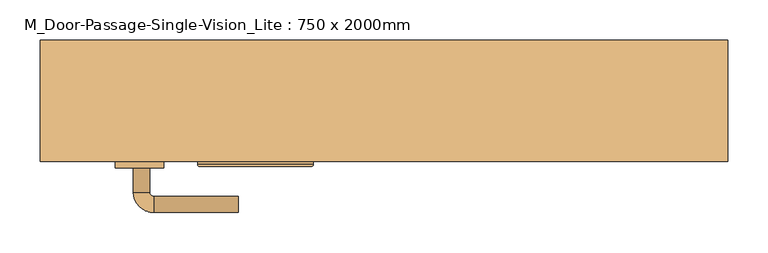
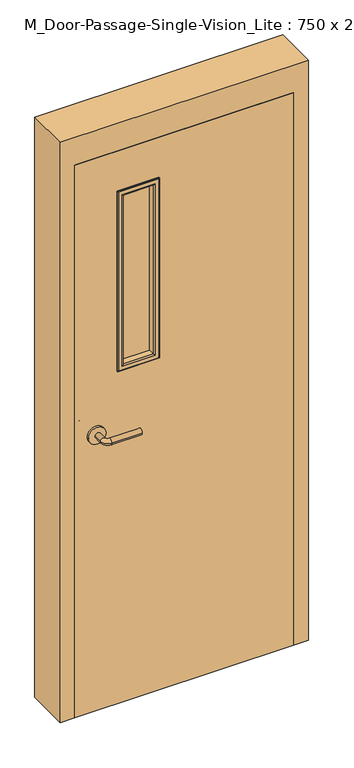
"""IFC4 building model written with IfcOpenShell, lengths in millimetres: door geometry, M_Door-Passage-Single-Vision_Lite : 750 x 2000mm."""

from ifc_helpers import new_model, si_unit, point, frame, frame_2d, origin, place, context, project, spatial, polyline, circle_curve, ellipse_curve, trimmed, segment, composite_curve, outline, extrude, faceted_brep, source, transform, mapped, element, save
from ifc_brep_helpers import plane_surface, cylinder_surface, revolved_surface, advanced_brep


def m_door_passage_single_vision_lite_750_x_2000mm_70ae5a51(model_context):
    return source(origin(), model_context, "Body", "SolidModel", [
        advanced_brep(
        [(-309.990625, -3.35, 1000.0), (-289.990625, -3.35, 1000.0), (-309.990625, 26.65, 1000.0), (-289.990625, 26.65, 1000.0), (-284.990625, 31.65, 1000.0), (-284.990625, 51.65, 1000.0), (-179.990625, 51.65, 1000.0), (-179.990625, 31.65, 1000.0)],
        [
            (0, 1, circle_curve(frame((-299.990625, -3.35, 1000.0), z_axis=(0.0, -1.0, 0.0), x_axis=(1.0, 0.0, 0.0)), 10.0)),
            (1, 0, circle_curve(frame((-299.990625, -3.35, 1000.0), z_axis=(0.0, -1.0, 0.0), x_axis=(1.0, 0.0, 0.0)), 10.0)),
            (0, 2),
            (2, 3, circle_curve(frame((-299.990625, 26.65, 1000.0), z_axis=(0.0, -1.0, 0.0), x_axis=(1.0, 0.0, 0.0)), 10.0)),
            (3, 1),
            (3, 2, circle_curve(frame((-299.990625, 26.65, 1000.0), z_axis=(0.0, -1.0, 0.0), x_axis=(1.0, 0.0, 0.0)), 10.0)),
            (4, 3, circle_curve(frame((-284.990625, 26.65, 1000.0), z_axis=(0.0, 0.0, 1.0), x_axis=(-1.0, 0.0, 0.0)), 5.0)),
            (2, 5, circle_curve(frame((-284.990625, 26.65, 1000.0), z_axis=(0.0, 0.0, -1.0), x_axis=(-1.0, 0.0, 0.0)), 25.0)),
            (5, 4, circle_curve(frame((-284.990625, 41.65, 1000.0), z_axis=(-1.0, 0.0, 0.0), x_axis=(0.0, -1.0, 0.0)), 10.0)),
            (4, 5, circle_curve(frame((-284.990625, 41.65, 1000.0), z_axis=(-1.0, 0.0, 0.0), x_axis=(0.0, -1.0, 0.0)), 10.0)),
            (6, 7, circle_curve(frame((-179.990625, 41.65, 1000.0), z_axis=(1.0, 0.0, 0.0), x_axis=(0.0, -1.0, 0.0)), 10.0)),
            (7, 6, circle_curve(frame((-179.990625, 41.65, 1000.0), z_axis=(1.0, 0.0, 0.0), x_axis=(0.0, -1.0, 0.0)), 10.0)),
            (5, 6),
            (7, 4),
        ],
        [
            plane_surface(frame((-299.990625, -3.35, 1000.0), z_axis=(0.0, -1.0, 0.0), x_axis=(0.0, 0.0, 1.0))),
            cylinder_surface(frame((-299.990625, -3.35, 1000.0), z_axis=(0.0, -1.0, 0.0), x_axis=(1.0, 0.0, 0.0)), 10.0),
            revolved_surface(trimmed(ellipse_curve(frame((-299.990625, 26.65, 1000.0), z_axis=(0.0, -1.0, 0.0), x_axis=(1.0, 0.0, 0.0)), 10.0, 10.0), [point((-309.990625, 26.65, 1000.0))], [point((-289.990625, 26.65, 1000.0))], True, "CARTESIAN"), (-284.990625, 26.65, 1000.0), (0.0, 0.0, -1.0)),
            revolved_surface(trimmed(ellipse_curve(frame((-299.990625, 26.65, 1000.0), z_axis=(0.0, -1.0, 0.0), x_axis=(1.0, 0.0, 0.0)), 10.0, 10.0), [point((-289.990625, 26.65, 1000.0))], [point((-309.990625, 26.65, 1000.0))], True, "CARTESIAN"), (-284.990625, 26.65, 1000.0), (0.0, 0.0, -1.0)),
            plane_surface(frame((-179.990625, 41.65, 1000.0), z_axis=(1.0, 0.0, 0.0), x_axis=(0.0, 0.0, 1.0))),
            cylinder_surface(frame((-284.990625, 41.65, 1000.0), z_axis=(-1.0, 0.0, 0.0), x_axis=(0.0, -1.0, 0.0)), 10.0),
        ],
        [
            (0, [[1, 2]]),
            (1, [[-1, 3, 4, 5]]),
            (1, [[-2, -5, 6, -3]]),
            (2, [[7, -4, 8, 9]]),
            (3, [[-8, -6, -7, 10]]),
            (4, [[11, 12]]),
            (5, [[-9, 13, -12, 14]]),
            (5, [[-10, -14, -11, -13]]),
        ],
    ),
        extrude(outline(composite_curve([segment(trimmed(circle_curve(frame_2d((1000.0, -302.490625)), 30.0), [point((1000.0, -332.490625))], [point((1000.0, -272.490625))], False, "CARTESIAN"), True, "CONTINUOUS"), segment(trimmed(circle_curve(frame_2d((1000.0, -302.490625)), 30.0), [point((1000.0, -272.490625))], [point((1000.0, -332.490625))], False, "CARTESIAN"), True, "CONTINUOUS")], self_intersect=False)), frame((0.0, -11.35, 0.0), z_axis=(0.0, 1.0, 0.0), x_axis=(0.0, 0.0, 1.0)), (0.0, 0.0, 1.0), 8.0),
        advanced_brep(
        [(-309.990625, -64.35, 1000.0), (-289.990625, -64.35, 1000.0), (-289.990625, -94.35, 1000.0), (-309.990625, -94.35, 1000.0), (-284.990625, -99.35, 1000.0), (-284.990625, -119.35, 1000.0), (-179.990625, -119.35, 1000.0), (-179.990625, -99.35, 1000.0)],
        [
            (0, 1, circle_curve(frame((-299.990625, -64.35, 1000.0), z_axis=(0.0, 1.0, 0.0), x_axis=(1.0, 0.0, 0.0)), 10.0)),
            (1, 0, circle_curve(frame((-299.990625, -64.35, 1000.0), z_axis=(0.0, 1.0, 0.0), x_axis=(1.0, 0.0, 0.0)), 10.0)),
            (1, 2),
            (2, 3, circle_curve(frame((-299.990625, -94.35, 1000.0), z_axis=(0.0, 1.0, 0.0), x_axis=(1.0, 0.0, 0.0)), 10.0)),
            (3, 0),
            (3, 2, circle_curve(frame((-299.990625, -94.35, 1000.0), z_axis=(0.0, 1.0, 0.0), x_axis=(1.0, 0.0, 0.0)), 10.0)),
            (4, 5, circle_curve(frame((-284.990625, -109.35, 1000.0), z_axis=(-1.0, 0.0, 0.0), x_axis=(0.0, 1.0, 0.0)), 10.0)),
            (5, 3, circle_curve(frame((-284.990625, -94.35, 1000.0), z_axis=(0.0, 0.0, -1.0), x_axis=(-1.0, 0.0, 0.0)), 25.0)),
            (2, 4, circle_curve(frame((-284.990625, -94.35, 1000.0), z_axis=(0.0, 0.0, 1.0), x_axis=(-1.0, 0.0, 0.0)), 5.0)),
            (5, 4, circle_curve(frame((-284.990625, -109.35, 1000.0), z_axis=(-1.0, 0.0, 0.0), x_axis=(0.0, 1.0, 0.0)), 10.0)),
            (6, 7, circle_curve(frame((-179.990625, -109.35, 1000.0), z_axis=(1.0, 0.0, 0.0), x_axis=(0.0, 1.0, 0.0)), 10.0)),
            (7, 6, circle_curve(frame((-179.990625, -109.35, 1000.0), z_axis=(1.0, 0.0, 0.0), x_axis=(0.0, 1.0, 0.0)), 10.0)),
            (4, 7),
            (6, 5),
        ],
        [
            plane_surface(frame((-299.990625, -64.35, 1000.0), z_axis=(0.0, 1.0, 0.0), x_axis=(0.0, 0.0, 1.0))),
            cylinder_surface(frame((-299.990625, -64.35, 1000.0), z_axis=(0.0, 1.0, 0.0), x_axis=(1.0, 0.0, 0.0)), 10.0),
            revolved_surface(trimmed(ellipse_curve(frame((-299.990625, -94.35, 1000.0), z_axis=(0.0, -1.0, 0.0), x_axis=(1.0, 0.0, 0.0)), 10.0, 10.0), [point((-309.990625, -94.35, 1000.0))], [point((-289.990625, -94.35, 1000.0))], True, "CARTESIAN"), (-284.990625, -94.35, 1000.0), (0.0, 0.0, -1.0)),
            revolved_surface(trimmed(ellipse_curve(frame((-299.990625, -94.35, 1000.0), z_axis=(0.0, -1.0, 0.0), x_axis=(1.0, 0.0, 0.0)), 10.0, 10.0), [point((-289.990625, -94.35, 1000.0))], [point((-309.990625, -94.35, 1000.0))], True, "CARTESIAN"), (-284.990625, -94.35, 1000.0), (0.0, 0.0, -1.0)),
            plane_surface(frame((-179.990625, -109.35, 1000.0), z_axis=(1.0, 0.0, 0.0), x_axis=(0.0, 0.0, 1.0))),
            cylinder_surface(frame((-284.990625, -109.35, 1000.0), z_axis=(-1.0, 0.0, 0.0), x_axis=(0.0, 1.0, 0.0)), 10.0),
        ],
        [
            (0, [[1, 2]]),
            (1, [[3, 4, 5, -2]]),
            (1, [[-5, 6, -3, -1]]),
            (2, [[7, 8, -4, 9]]),
            (3, [[10, -9, -6, -8]]),
            (4, [[11, 12]]),
            (5, [[13, -11, 14, -7]]),
            (5, [[-14, -12, -13, -10]]),
        ],
    ),
        extrude(outline(composite_curve([segment(trimmed(circle_curve(frame_2d((1000.0, -302.490625)), 30.0), [point((1000.0, -332.490625))], [point((1000.0, -272.490625))], False, "CARTESIAN"), True, "CONTINUOUS"), segment(trimmed(circle_curve(frame_2d((1000.0, -302.490625)), 30.0), [point((1000.0, -272.490625))], [point((1000.0, -332.490625))], False, "CARTESIAN"), True, "CONTINUOUS")], self_intersect=False)), frame((0.0, -64.35, 0.0), z_axis=(0.0, 1.0, 0.0), x_axis=(0.0, 0.0, 1.0)), (0.0, 0.0, 1.0), 8.0),
        extrude(outline(polyline([(2000.0, -375.0), (0.0, -375.0), (0.0, 375.0), (2000.0, 375.0), (2000.0, -375.0)]), holes=[polyline([(1847.6, -222.6), (1847.6, -95.6), (1212.6, -95.6), (1212.6, -222.6), (1847.6, -222.6)])]), frame((0.0, -56.35, 0.0), z_axis=(0.0, 1.0, 0.0), x_axis=(0.0, 0.0, 1.0)), (0.0, 0.0, 1.0), 45.0),
        faceted_brep([(375.0, -6.5875, 0.0), (359.125, -6.5875, 0.0), (359.125, 44.4375, 0.0), (375.0, 44.4375, 0.0), (375.0, 93.65, 0.0), (425.0, 93.65, 0.0), (425.0, -56.35, 0.0), (375.0, -56.35, 0.0), (375.0, -56.35, 2000.0), (375.0, -6.5875, 2000.0), (425.0, -56.35, 2100.0), (-425.0, -56.35, 2100.0), (-425.0, -56.35, 0.0), (-375.0, -56.35, 0.0), (-375.0, -56.35, 2000.0), (425.0, 93.65, 2100.0), (375.0, 93.65, 2000.0), (-375.0, 93.65, 2000.0), (-375.0, 93.65, 0.0), (-425.0, 93.65, 0.0), (-425.0, 93.65, 2100.0), (375.0, 44.4375, 2000.0), (359.125, 44.4375, 1984.125), (-359.125, 44.4375, 1984.125), (-359.125, 44.4375, 0.0), (-375.0, 44.4375, 0.0), (-375.0, 44.4375, 2000.0), (359.125, -6.5875, 1984.125), (-375.0, -6.5875, 2000.0), (-375.0, -6.5875, 0.0), (-359.125, -6.5875, 0.0), (-359.125, -6.5875, 1984.125)], [[[0, 1, 2, 3, 4, 5, 6, 7]], [[7, 8, 9, 0]], [[6, 10, 11, 12, 13, 14, 8, 7]], [[5, 15, 10, 6]], [[4, 16, 17, 18, 19, 20, 15, 5]], [[3, 21, 16, 4]], [[2, 22, 23, 24, 25, 26, 21, 3]], [[1, 27, 22, 2]], [[0, 9, 28, 29, 30, 31, 27, 1]], [[8, 14, 28, 9]], [[16, 21, 26, 17]], [[22, 27, 31, 23]], [[12, 19, 18, 25, 24, 30, 29, 13]], [[13, 29, 28, 14]], [[11, 20, 19, 12]], [[17, 26, 25, 18]], [[23, 31, 30, 24]], [[15, 20, 11, 10]]]),
        extrude(outline(polyline([(-95.6, -31.35), (-95.6, -36.35), (-222.6, -36.35), (-222.6, -31.35), (-95.6, -31.35)])), frame((0.0, 0.0, 1212.6), z_axis=(0.0, 0.0, 1.0), x_axis=(1.0, 0.0, 0.0)), (0.0, 0.0, 1.0), 635.0),
        advanced_brep(
        [(-222.6, -36.35, 1847.6), (-222.6, -36.35, 1212.6), (-222.6, -56.35, 1212.6), (-222.6, -56.35, 1847.6), (-210.6, -57.35, 1835.6), (-210.6, -57.35, 1224.6), (-210.6, -36.35, 1224.6), (-210.6, -36.35, 1835.6), (-215.6, -62.35, 1840.6), (-215.6, -62.35, 1219.6), (-230.6, -60.35, 1855.6), (-230.6, -60.35, 1204.6), (-228.6, -62.35, 1206.6), (-228.6, -62.35, 1853.6), (-230.6, -56.35, 1855.6), (-230.6, -56.35, 1204.6), (-95.6, -36.35, 1212.6), (-95.6, -56.35, 1212.6), (-107.6, -57.35, 1224.6), (-107.6, -36.35, 1224.6), (-102.6, -62.35, 1219.6), (-87.6, -60.35, 1204.6), (-89.6, -62.35, 1206.6), (-87.6, -56.35, 1204.6), (-95.6, -36.35, 1847.6), (-95.6, -56.35, 1847.6), (-107.6, -57.35, 1835.6), (-107.6, -36.35, 1835.6), (-102.6, -62.35, 1840.6), (-87.6, -60.35, 1855.6), (-89.6, -62.35, 1853.6), (-87.6, -56.35, 1855.6)],
        [
            (0, 1),
            (1, 2),
            (2, 3),
            (3, 0),
            (4, 5),
            (5, 6),
            (6, 7),
            (7, 4),
            (8, 9),
            (9, 5, ellipse_curve(frame((-215.6, -57.35, 1219.6), z_axis=(-0.7071067811865475, 0.0, 0.7071067811865475), x_axis=(0.7071067811865474, 0.0, 0.7071067811865476)), 7.0710678, 5.0)),
            (4, 8, ellipse_curve(frame((-215.6, -57.35, 1840.6), z_axis=(-0.7071067811865475, 0.0, -0.7071067811865475), x_axis=(-0.7071067811865474, 0.0, 0.7071067811865476)), 7.0710678, 5.0)),
            (10, 11),
            (11, 12, ellipse_curve(frame((-228.6, -60.35, 1206.6), z_axis=(-0.7071067811865475, 0.0, 0.7071067811865475), x_axis=(0.7071067811865474, 0.0, 0.7071067811865476)), 2.8284271, 2.0)),
            (12, 13),
            (13, 10, ellipse_curve(frame((-228.6, -60.35, 1853.6), z_axis=(-0.7071067811865475, 0.0, -0.7071067811865475), x_axis=(-0.7071067811865474, 0.0, 0.7071067811865476)), 2.8284271, 2.0)),
            (14, 15),
            (15, 11),
            (10, 14),
            (1, 16),
            (16, 17),
            (17, 2),
            (5, 18),
            (18, 19),
            (19, 6),
            (9, 20),
            (20, 18, ellipse_curve(frame((-102.6, -57.35, 1219.6), z_axis=(-0.7071067811865475, 0.0, -0.7071067811865475), x_axis=(-0.7071067811865476, 0.0, 0.7071067811865474)), 7.0710678, 5.0)),
            (11, 21),
            (21, 22, ellipse_curve(frame((-89.6, -60.35, 1206.6), z_axis=(-0.7071067811865475, 0.0, -0.7071067811865475), x_axis=(-0.7071067811865476, 0.0, 0.7071067811865474)), 2.8284271, 2.0)),
            (22, 12),
            (15, 23),
            (23, 21),
            (16, 24),
            (24, 25),
            (25, 17),
            (18, 26),
            (26, 27),
            (27, 19),
            (20, 28),
            (28, 26, ellipse_curve(frame((-102.6, -57.35, 1840.6), z_axis=(0.7071067811865475, 0.0, -0.7071067811865475), x_axis=(-0.7071067811865474, 0.0, -0.7071067811865476)), 7.0710678, 5.0)),
            (21, 29),
            (29, 30, ellipse_curve(frame((-89.6, -60.35, 1853.6), z_axis=(0.7071067811865475, 0.0, -0.7071067811865475), x_axis=(-0.7071067811865474, 0.0, -0.7071067811865476)), 2.8284271, 2.0)),
            (30, 22),
            (23, 31),
            (31, 29),
            (14, 31),
            (25, 3),
            (24, 0),
            (27, 7),
            (26, 4),
            (28, 8),
            (30, 13),
            (29, 10),
        ],
        [
            plane_surface(frame((-222.6, -56.35, 1847.6), z_axis=(-1.0, 0.0, 0.0), x_axis=(0.0, 0.0, -1.0))),
            plane_surface(frame((-210.6, -36.35, 1835.6), z_axis=(1.0, 0.0, 0.0), x_axis=(0.0, 0.0, -1.0))),
            cylinder_surface(frame((-215.6, -57.35, 1847.6), z_axis=(0.0, 0.0, 1.0), x_axis=(-1.0, 0.0, 0.0)), 5.0),
            cylinder_surface(frame((-228.6, -60.35, 1847.6), z_axis=(0.0, 0.0, 1.0), x_axis=(-1.0, 0.0, 0.0)), 2.0),
            plane_surface(frame((-230.6, -60.35, 1855.6), z_axis=(-1.0, 0.0, 0.0), x_axis=(0.0, 0.0, -1.0))),
            plane_surface(frame((-222.6, -56.35, 1212.6), z_axis=(0.0, 0.0, -1.0), x_axis=(1.0, 0.0, 0.0))),
            plane_surface(frame((-210.6, -36.35, 1224.6), z_axis=(0.0, 0.0, 1.0), x_axis=(1.0, 0.0, 0.0))),
            cylinder_surface(frame((-222.6, -57.35, 1219.6), z_axis=(-1.0, 0.0, 0.0), x_axis=(0.0, 0.0, -1.0)), 5.0),
            cylinder_surface(frame((-222.6, -60.35, 1206.6), z_axis=(-1.0, 0.0, 0.0), x_axis=(0.0, 0.0, -1.0)), 2.0),
            plane_surface(frame((-230.6, -60.35, 1204.6), z_axis=(0.0, 0.0, -1.0), x_axis=(1.0, 0.0, 0.0))),
            plane_surface(frame((-95.6, -56.35, 1212.6), z_axis=(1.0, 0.0, 0.0), x_axis=(0.0, 0.0, 1.0))),
            plane_surface(frame((-107.6, -36.35, 1224.6), z_axis=(-1.0, 0.0, 0.0), x_axis=(0.0, 0.0, 1.0))),
            cylinder_surface(frame((-102.6, -57.35, 1212.6), z_axis=(0.0, 0.0, -1.0), x_axis=(1.0, 0.0, 0.0)), 5.0),
            cylinder_surface(frame((-89.6, -60.35, 1212.6), z_axis=(0.0, 0.0, -1.0), x_axis=(1.0, 0.0, 0.0)), 2.0),
            plane_surface(frame((-87.6, -60.35, 1204.6), z_axis=(1.0, 0.0, 0.0), x_axis=(0.0, 0.0, 1.0))),
            plane_surface(frame((-87.6, -56.35, 1855.6), z_axis=(0.0, 1.0, 0.0), x_axis=(-1.0, 0.0, 0.0))),
            plane_surface(frame((-95.6, -56.35, 1847.6), z_axis=(0.0, 0.0, 1.0), x_axis=(-1.0, 0.0, 0.0))),
            plane_surface(frame((-95.6, -36.35, 1847.6), z_axis=(0.0, 1.0, 0.0), x_axis=(-1.0, 0.0, 0.0))),
            plane_surface(frame((-107.6, -36.35, 1835.6), z_axis=(0.0, 0.0, -1.0), x_axis=(-1.0, 0.0, 0.0))),
            cylinder_surface(frame((-95.6, -57.35, 1840.6), z_axis=(1.0, 0.0, 0.0), x_axis=(0.0, 0.0, 1.0)), 5.0),
            plane_surface(frame((-102.6, -62.35, 1840.6), z_axis=(0.0, -1.0, 0.0), x_axis=(-1.0, 0.0, 0.0))),
            cylinder_surface(frame((-95.6, -60.35, 1853.6), z_axis=(1.0, 0.0, 0.0), x_axis=(0.0, 0.0, 1.0)), 2.0),
            plane_surface(frame((-87.6, -60.35, 1855.6), z_axis=(0.0, 0.0, 1.0), x_axis=(-1.0, 0.0, 0.0))),
        ],
        [
            (0, [[1, 2, 3, 4]]),
            (1, [[5, 6, 7, 8]]),
            (2, [[9, 10, -5, 11]]),
            (3, [[12, 13, 14, 15]]),
            (4, [[16, 17, -12, 18]]),
            (5, [[19, 20, 21, -2]]),
            (6, [[22, 23, 24, -6]]),
            (7, [[25, 26, -22, -10]]),
            (8, [[27, 28, 29, -13]]),
            (9, [[30, 31, -27, -17]]),
            (10, [[32, 33, 34, -20]]),
            (11, [[35, 36, 37, -23]]),
            (12, [[38, 39, -35, -26]]),
            (13, [[40, 41, 42, -28]]),
            (14, [[43, 44, -40, -31]]),
            (15, [[-16, 45, -43, -30], [-3, -21, -34, 46]]),
            (16, [[47, -4, -46, -33]]),
            (17, [[-1, -47, -32, -19], [-7, -24, -37, 48]]),
            (18, [[49, -8, -48, -36]]),
            (19, [[50, -11, -49, -39]]),
            (20, [[-14, -29, -42, 51], [-9, -50, -38, -25]]),
            (21, [[52, -15, -51, -41]]),
            (22, [[-45, -18, -52, -44]]),
        ],
    ),
        advanced_brep(
        [(-222.6, -31.35, 1212.6), (-222.6, -31.35, 1847.6), (-222.6, -11.35, 1847.6), (-222.6, -11.35, 1212.6), (-210.6, -10.35, 1224.6), (-210.6, -10.35, 1835.6), (-210.6, -31.35, 1835.6), (-210.6, -31.35, 1224.6), (-215.6, -5.35, 1219.6), (-215.6, -5.35, 1840.6), (-230.6, -7.35, 1204.6), (-230.6, -7.35, 1855.6), (-228.6, -5.35, 1853.6), (-228.6, -5.35, 1206.6), (-230.6, -11.35, 1204.6), (-230.6, -11.35, 1855.6), (-95.6, -31.35, 1847.6), (-95.6, -11.35, 1847.6), (-107.6, -10.35, 1835.6), (-107.6, -31.35, 1835.6), (-102.6, -5.35, 1840.6), (-87.6, -7.35, 1855.6), (-89.6, -5.35, 1853.6), (-87.6, -11.35, 1855.6), (-95.6, -31.35, 1212.6), (-95.6, -11.35, 1212.6), (-107.6, -10.35, 1224.6), (-107.6, -31.35, 1224.6), (-102.6, -5.35, 1219.6), (-87.6, -7.35, 1204.6), (-89.6, -5.35, 1206.6), (-87.6, -11.35, 1204.6)],
        [
            (0, 1),
            (1, 2),
            (2, 3),
            (3, 0),
            (4, 5),
            (5, 6),
            (6, 7),
            (7, 4),
            (8, 9),
            (9, 5, ellipse_curve(frame((-215.6, -10.35, 1840.6), z_axis=(-0.7071067811865475, 0.0, -0.7071067811865475), x_axis=(0.7071067811865474, 0.0, -0.7071067811865476)), 7.0710678, 5.0)),
            (4, 8, ellipse_curve(frame((-215.6, -10.35, 1219.6), z_axis=(-0.7071067811865475, 0.0, 0.7071067811865475), x_axis=(-0.7071067811865474, 0.0, -0.7071067811865476)), 7.0710678, 5.0)),
            (10, 11),
            (11, 12, ellipse_curve(frame((-228.6, -7.35, 1853.6), z_axis=(-0.7071067811865475, 0.0, -0.7071067811865475), x_axis=(0.7071067811865474, 0.0, -0.7071067811865476)), 2.8284271, 2.0)),
            (12, 13),
            (13, 10, ellipse_curve(frame((-228.6, -7.35, 1206.6), z_axis=(-0.7071067811865475, 0.0, 0.7071067811865475), x_axis=(-0.7071067811865474, 0.0, -0.7071067811865476)), 2.8284271, 2.0)),
            (14, 15),
            (15, 11),
            (10, 14),
            (1, 16),
            (16, 17),
            (17, 2),
            (5, 18),
            (18, 19),
            (19, 6),
            (9, 20),
            (20, 18, ellipse_curve(frame((-102.6, -10.35, 1840.6), z_axis=(-0.7071067811865475, 0.0, 0.7071067811865475), x_axis=(-0.7071067811865476, 0.0, -0.7071067811865474)), 7.0710678, 5.0)),
            (11, 21),
            (21, 22, ellipse_curve(frame((-89.6, -7.35, 1853.6), z_axis=(-0.7071067811865475, 0.0, 0.7071067811865475), x_axis=(-0.7071067811865476, 0.0, -0.7071067811865474)), 2.8284271, 2.0)),
            (22, 12),
            (15, 23),
            (23, 21),
            (16, 24),
            (24, 25),
            (25, 17),
            (18, 26),
            (26, 27),
            (27, 19),
            (20, 28),
            (28, 26, ellipse_curve(frame((-102.6, -10.35, 1219.6), z_axis=(0.7071067811865475, 0.0, 0.7071067811865475), x_axis=(-0.7071067811865474, 0.0, 0.7071067811865476)), 7.0710678, 5.0)),
            (21, 29),
            (29, 30, ellipse_curve(frame((-89.6, -7.35, 1206.6), z_axis=(0.7071067811865475, 0.0, 0.7071067811865475), x_axis=(-0.7071067811865474, 0.0, 0.7071067811865476)), 2.8284271, 2.0)),
            (30, 22),
            (23, 31),
            (31, 29),
            (14, 31),
            (25, 3),
            (24, 0),
            (27, 7),
            (26, 4),
            (28, 8),
            (30, 13),
            (29, 10),
        ],
        [
            plane_surface(frame((-222.6, -11.35, 1212.6), z_axis=(-1.0, 0.0, 0.0), x_axis=(0.0, 0.0, 1.0))),
            plane_surface(frame((-210.6, -31.35, 1224.6), z_axis=(1.0, 0.0, 0.0), x_axis=(0.0, 0.0, 1.0))),
            cylinder_surface(frame((-215.6, -10.35, 1212.6), z_axis=(0.0, 0.0, -1.0), x_axis=(-1.0, 0.0, 0.0)), 5.0),
            cylinder_surface(frame((-228.6, -7.35, 1212.6), z_axis=(0.0, 0.0, -1.0), x_axis=(-1.0, 0.0, 0.0)), 2.0),
            plane_surface(frame((-230.6, -7.35, 1204.6), z_axis=(-1.0, 0.0, 0.0), x_axis=(0.0, 0.0, 1.0))),
            plane_surface(frame((-222.6, -11.35, 1847.6), z_axis=(0.0, 0.0, 1.0), x_axis=(1.0, 0.0, 0.0))),
            plane_surface(frame((-210.6, -31.35, 1835.6), z_axis=(0.0, 0.0, -1.0), x_axis=(1.0, 0.0, 0.0))),
            cylinder_surface(frame((-222.6, -10.35, 1840.6), z_axis=(-1.0, 0.0, 0.0), x_axis=(0.0, 0.0, 1.0)), 5.0),
            cylinder_surface(frame((-222.6, -7.35, 1853.6), z_axis=(-1.0, 0.0, 0.0), x_axis=(0.0, 0.0, 1.0)), 2.0),
            plane_surface(frame((-230.6, -7.35, 1855.6), z_axis=(0.0, 0.0, 1.0), x_axis=(1.0, 0.0, 0.0))),
            plane_surface(frame((-95.6, -11.35, 1847.6), z_axis=(1.0, 0.0, 0.0), x_axis=(0.0, 0.0, -1.0))),
            plane_surface(frame((-107.6, -31.35, 1835.6), z_axis=(-1.0, 0.0, 0.0), x_axis=(0.0, 0.0, -1.0))),
            cylinder_surface(frame((-102.6, -10.35, 1847.6), z_axis=(0.0, 0.0, 1.0), x_axis=(1.0, 0.0, 0.0)), 5.0),
            cylinder_surface(frame((-89.6, -7.35, 1847.6), z_axis=(0.0, 0.0, 1.0), x_axis=(1.0, 0.0, 0.0)), 2.0),
            plane_surface(frame((-87.6, -7.35, 1855.6), z_axis=(1.0, 0.0, 0.0), x_axis=(0.0, 0.0, -1.0))),
            plane_surface(frame((-87.6, -11.35, 1204.6), z_axis=(0.0, -1.0, 0.0), x_axis=(-1.0, 0.0, 0.0))),
            plane_surface(frame((-95.6, -11.35, 1212.6), z_axis=(0.0, 0.0, -1.0), x_axis=(-1.0, 0.0, 0.0))),
            plane_surface(frame((-95.6, -31.35, 1212.6), z_axis=(0.0, -1.0, 0.0), x_axis=(-1.0, 0.0, 0.0))),
            plane_surface(frame((-107.6, -31.35, 1224.6), z_axis=(0.0, 0.0, 1.0), x_axis=(-1.0, 0.0, 0.0))),
            cylinder_surface(frame((-95.6, -10.35, 1219.6), z_axis=(1.0, 0.0, 0.0), x_axis=(0.0, 0.0, -1.0)), 5.0),
            plane_surface(frame((-102.6, -5.35, 1219.6), z_axis=(0.0, 1.0, 0.0), x_axis=(-1.0, 0.0, 0.0))),
            cylinder_surface(frame((-95.6, -7.35, 1206.6), z_axis=(1.0, 0.0, 0.0), x_axis=(0.0, 0.0, -1.0)), 2.0),
            plane_surface(frame((-87.6, -7.35, 1204.6), z_axis=(0.0, 0.0, -1.0), x_axis=(-1.0, 0.0, 0.0))),
        ],
        [
            (0, [[1, 2, 3, 4]]),
            (1, [[5, 6, 7, 8]]),
            (2, [[9, 10, -5, 11]]),
            (3, [[12, 13, 14, 15]]),
            (4, [[16, 17, -12, 18]]),
            (5, [[19, 20, 21, -2]]),
            (6, [[22, 23, 24, -6]]),
            (7, [[25, 26, -22, -10]]),
            (8, [[27, 28, 29, -13]]),
            (9, [[30, 31, -27, -17]]),
            (10, [[32, 33, 34, -20]]),
            (11, [[35, 36, 37, -23]]),
            (12, [[38, 39, -35, -26]]),
            (13, [[40, 41, 42, -28]]),
            (14, [[43, 44, -40, -31]]),
            (15, [[-16, 45, -43, -30], [-3, -21, -34, 46]]),
            (16, [[47, -4, -46, -33]]),
            (17, [[-1, -47, -32, -19], [-7, -24, -37, 48]]),
            (18, [[49, -8, -48, -36]]),
            (19, [[50, -11, -49, -39]]),
            (20, [[-14, -29, -42, 51], [-9, -50, -38, -25]]),
            (21, [[52, -15, -51, -41]]),
            (22, [[-45, -18, -52, -44]]),
        ],
    ),
    ])


if __name__ == "__main__":
    model = new_model("IFC4")
    model_context = context("Model", 3, world=origin())
    ifc_project = project(units=[si_unit("LENGTHUNIT", "METRE", prefix="MILLI")], contexts=[model_context])
    site = spatial("IfcSite", under=ifc_project)
    building = spatial("IfcBuilding", under=site)
    placement = place(None, origin())
    m_door_passage_single_vision_lite_750_x_2000mm_shape = m_door_passage_single_vision_lite_750_x_2000mm_70ae5a51(model_context)
    element("IfcDoor", 1, ObjectType="M_Door-Passage-Single-Vision_Lite : 750 x 2000mm", at=placement, inside=building, context=model_context, shape_type="MappedRepresentation", body=[
        mapped(m_door_passage_single_vision_lite_750_x_2000mm_shape, transform((0.0, 0.0, 0.0), x_axis=(1.0, 0.0, 0.0), y_axis=(0.0, 1.0, 0.0), z_axis=(0.0, 0.0, 1.0))),
    ])
    save(model, "model.ifc")

# Revit data of these elements
# Type "M_Door-Passage-Single-Vision_Lite : 750 x 2000mm"
#   Type Mark = "42"
#   Analytic Construction = "Wooden"
#   Thickness = 45 mm
#   Thermal Resistance (R) = 0.455703 (m²·K)/W
#   Swing Angle [instance default] = 90.00°
#   Strike Height = 1000 mm
#   Rough Width [instance default] = 850 mm
#   Rough Height [instance default] = 2100 mm
#   MFOpeningHeight [instance default] = 100 mm
#   MFOpeningWidth [instance default] = 100 mm
#   Inset Calculate [instance default] = 105 mm
#   Masonry Inset [instance default] = 25 mm
#   Height = 2000 mm
#   Width = 750 mm
#   Heat Transfer Coefficient (U) = 2.19465 W/(m²·K)
#   Masonry Frame Depth = 150 mm
#   Masonry Frame [instance default] = yes
#   Function = 1
#   Dry Wall Frame [instance default] = no
#   Panel Material = Wood - Birch
#   Glazing = Glass
#   Glass Stop Material = Metal - Paint Finish - Grey
#   Frame Material = Metal - Paint Finish - Grey
#   Door Handle Material = Aluminum
#   Visual Light Transmittance = 0
#   Solar Heat Gain Coefficient = 0
#   Wall Closure = (empty or 0)
# Element 1 (IfcDoor, "M_Door-Passage-Single-Vision_Lite : 750 x 2000mm")
#   Materials on its faces: "Metal - Paint Finish - Grey", "Aluminum", "Wood - Birch", "Glass"
# Materials
#   "Wood - Birch": class "Wood", colour RGB 173 132 96, transparency 0, Cost = 0
#   "Glass": class "Glass", colour RGB 245 245 243, transparency 1, Description = "Soda Lime Glass", Cost = 0
#   "Metal - Paint Finish - Grey": class "Paint", colour RGB 178 178 178, transparency 0, Cost = 0
#   "Aluminum": class "Metal", colour RGB 244 245 246, transparency 0, Description = "Aluminum 6061", Cost = 0
